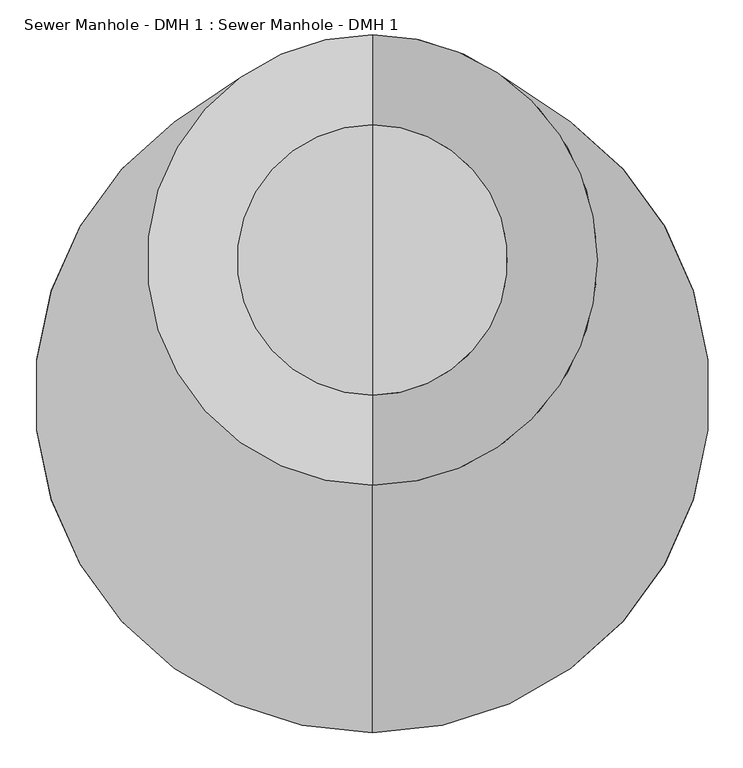
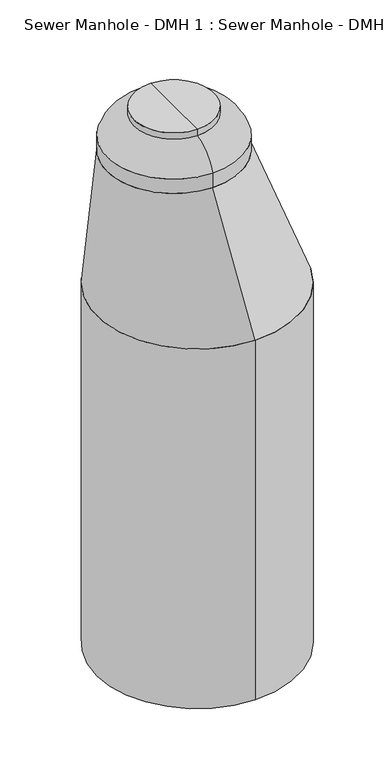
"""IFC4 building model written with IfcOpenShell, lengths in millimetres: proxy geometry, Sewer Manhole - DMH 1 : Sewer Manhole - DMH 1."""

from ifc_helpers import new_model, si_unit, point, frame, origin, place, context, project, spatial, circle_curve, ellipse_curve, trimmed, source, transform, mapped, element, save
from ifc_brep_helpers import plane_surface, cylinder_surface, revolved_surface, spline_surface, advanced_brep


def sewer_manhole_dmh_1_sewer_manhole_dmh_1_3a11640a(model_context):
    return source(origin(), model_context, "Body", "AdvancedBrep", [
        advanced_brep(
        [(0.0, -203.2, 3771.1270774), (0.0, 812.8, 3771.1270774), (0.0, -762.0, 2885.44), (0.0, 762.0, 2885.44)],
        [
            (0, 1, circle_curve(frame((0.0, 304.8, 3771.1270774), z_axis=(0.0, 0.0, 1.0), x_axis=(0.0, 1.0, 0.0)), 508.0)),
            (1, 0, circle_curve(frame((0.0, 304.8, 3771.1270774), z_axis=(0.0, 0.0, 1.0), x_axis=(0.0, 1.0, 0.0)), 508.0)),
            (2, 3, circle_curve(frame((0.0, 0.0, 2885.44), z_axis=(0.0, 0.0, -1.0), x_axis=(0.0, 1.0, 0.0)), 762.0)),
            (3, 2, circle_curve(frame((0.0, 0.0, 2885.44), z_axis=(0.0, 0.0, -1.0), x_axis=(0.0, 1.0, 0.0)), 762.0)),
            (3, 1),
            (0, 2),
        ],
        [
            plane_surface(frame((0.0, 304.8, 3771.1270774), z_axis=(0.0, 0.0, 1.0), x_axis=(1.0, 0.0, 0.0))),
            plane_surface(frame((0.0, 0.0, 2885.44), z_axis=(0.0, 0.0, -1.0), x_axis=(1.0, 0.0, 0.0))),
            spline_surface(2, 1, [[(0.0, -762.0, 2885.44), (0.0, -203.2, 3771.1270774)], [(762.0, -762.0, 2885.44), (508.0, -203.2, 3771.1270774)], [(762.0, 0.0, 2885.44), (508.0, 304.8, 3771.1270774)], [(762.0, 762.0, 2885.44), (508.0, 812.8, 3771.1270774)], [(0.0, 762.0, 2885.44), (0.0, 812.8, 3771.1270774)]], [3, 2, 3], [2, 2], [0.0, 1.0, 2.0], [0.0, 1.0], weights=[[1.0, 1.0], [0.7071067811865476, 0.7071067811865476], [1.0, 1.0], [0.7071067811865476, 0.7071067811865476], [1.0, 1.0]]),
            spline_surface(2, 1, [[(0.0, 762.0, 2885.44), (0.0, 812.8, 3771.1270774)], [(-762.0, 762.0, 2885.44), (-507.99999999999994, 812.8, 3771.1270774)], [(-762.0, 0.0, 2885.44), (-507.99999999999994, 304.8, 3771.1270774)], [(-762.0, -762.0, 2885.44), (-507.99999999999994, -203.19999999999993, 3771.1270774)], [(0.0, -762.0, 2885.44), (0.0, -203.2, 3771.1270774)]], [3, 2, 3], [2, 2], [0.0, 1.0, 2.0], [0.0, 1.0], weights=[[1.0, 1.0], [0.7071067811865476, 0.7071067811865476], [1.0, 1.0], [0.7071067811865476, 0.7071067811865476], [1.0, 1.0]]),
        ],
        [
            (0, [[1, 2]]),
            (1, [[3, 4]]),
            (2, [[-4, 5, -1, 6]]),
            (3, [[-3, -6, -2, -5]]),
        ],
    ),
        advanced_brep(
        [(0.0, -203.2, 3771.1270774), (0.0, 812.8, 3771.1270774), (0.0, 304.8, 3771.1270774), (0.0, -203.2, 3886.2), (0.0, 812.8, 3886.2), (0.0, 0.0, 4064.0), (0.0, 609.6, 4064.0), (0.0, 0.0, 4114.8), (0.0, 609.6, 4114.8), (0.0, 304.8, 4114.8)],
        [
            (0, 1, circle_curve(frame((0.0, 304.8, 3771.1270774), z_axis=(0.0, 0.0, -1.0), x_axis=(0.0, 1.0, 0.0)), 508.0)),
            (1, 2),
            (2, 0),
            (1, 0, circle_curve(frame((0.0, 304.8, 3771.1270774), z_axis=(0.0, 0.0, -1.0), x_axis=(0.0, 1.0, 0.0)), 508.0)),
            (3, 4, circle_curve(frame((0.0, 304.8, 3886.2), z_axis=(0.0, 0.0, -1.0), x_axis=(0.0, 1.0, 0.0)), 508.0)),
            (4, 1),
            (0, 3),
            (4, 3, circle_curve(frame((0.0, 304.8, 3886.2), z_axis=(0.0, 0.0, -1.0), x_axis=(0.0, 1.0, 0.0)), 508.0)),
            (5, 6, circle_curve(frame((0.0, 304.8, 4064.0), z_axis=(0.0, 0.0, -1.0), x_axis=(0.0, 1.0, 0.0)), 304.8)),
            (6, 4, circle_curve(frame((0.0, 564.4539436, 3807.3902213), z_axis=(-1.0, 0.0, 0.0), x_axis=(0.0, -1.0, 0.0)), 260.550849)),
            (3, 5, circle_curve(frame((0.0, 45.1460564, 3807.3902213), z_axis=(-1.0, 0.0, 0.0), x_axis=(0.0, 1.0, 0.0)), 260.550849)),
            (6, 5, circle_curve(frame((0.0, 304.8, 4064.0), z_axis=(0.0, 0.0, -1.0), x_axis=(0.0, 1.0, 0.0)), 304.8)),
            (7, 8, circle_curve(frame((0.0, 304.8, 4114.8), z_axis=(0.0, 0.0, -1.0), x_axis=(0.0, 1.0, 0.0)), 304.8)),
            (8, 6),
            (5, 7),
            (8, 7, circle_curve(frame((0.0, 304.8, 4114.8), z_axis=(0.0, 0.0, -1.0), x_axis=(0.0, 1.0, 0.0)), 304.8)),
            (9, 8),
            (7, 9),
        ],
        [
            plane_surface(frame((0.0, 304.8, 3771.1270774), z_axis=(0.0, 0.0, -1.0), x_axis=(0.0, 1.0, 0.0))),
            cylinder_surface(frame((0.0, 304.8, 3835.4), z_axis=(0.0, 0.0, 1.0), x_axis=(0.0, 1.0, 0.0)), 508.0),
            revolved_surface(trimmed(ellipse_curve(frame((0.0, 564.4539436, 3807.3902213), z_axis=(1.0, 0.0, 0.0), x_axis=(0.0, -1.0, 0.0)), 260.550849, 260.550849), [point((0.0, 812.8, 3886.2))], [point((0.0, 609.6, 4064.0))], True, "CARTESIAN"), (0.0, 304.8, 3835.4), (0.0, 0.0, 1.0)),
            cylinder_surface(frame((0.0, 304.8, 3835.4), z_axis=(0.0, 0.0, 1.0), x_axis=(0.0, 1.0, 0.0)), 304.8),
            plane_surface(frame((0.0, 304.8, 4114.8), z_axis=(0.0, 0.0, 1.0), x_axis=(0.0, 1.0, 0.0))),
        ],
        [
            (0, [[1, 2, 3]]),
            (0, [[4, -3, -2]]),
            (1, [[5, 6, -1, 7]]),
            (1, [[8, -7, -4, -6]]),
            (2, [[9, 10, -5, 11]]),
            (2, [[12, -11, -8, -10]]),
            (3, [[13, 14, -9, 15]]),
            (3, [[16, -15, -12, -14]]),
            (4, [[17, -13, 18]]),
            (4, [[-18, -16, -17]]),
        ],
    ),
        advanced_brep(
        [(0.0, -762.0, 2885.44), (0.0, 762.0, 2885.44), (0.0, 762.0, 0.0), (0.0, -762.0, 0.0), (0.0, 0.0, 0.0), (0.0, 0.0, 2885.44)],
        [
            (0, 1, circle_curve(frame((0.0, 0.0, 2885.44), z_axis=(0.0, 0.0, -1.0), x_axis=(0.0, 1.0, 0.0)), 762.0)),
            (1, 2),
            (2, 3, circle_curve(frame((0.0, 0.0, 0.0), z_axis=(0.0, 0.0, 1.0), x_axis=(0.0, 1.0, 0.0)), 762.0)),
            (3, 0),
            (1, 0, circle_curve(frame((0.0, 0.0, 2885.44), z_axis=(0.0, 0.0, -1.0), x_axis=(0.0, 1.0, 0.0)), 762.0)),
            (3, 2, circle_curve(frame((0.0, 0.0, 0.0), z_axis=(0.0, 0.0, 1.0), x_axis=(0.0, 1.0, 0.0)), 762.0)),
            (2, 4),
            (4, 3),
            (5, 1),
            (0, 5),
        ],
        [
            cylinder_surface(frame((0.0, 0.0, 457.2), z_axis=(0.0, 0.0, 1.0), x_axis=(0.0, 1.0, 0.0)), 762.0),
            plane_surface(frame((0.0, 0.0, 0.0), z_axis=(0.0, 0.0, -1.0), x_axis=(0.0, 1.0, 0.0))),
            plane_surface(frame((0.0, 0.0, 2885.44), z_axis=(0.0, 0.0, 1.0), x_axis=(0.0, 1.0, 0.0))),
        ],
        [
            (0, [[1, 2, 3, 4]]),
            (0, [[5, -4, 6, -2]]),
            (1, [[-3, 7, 8]]),
            (1, [[-6, -8, -7]]),
            (2, [[9, -1, 10]]),
            (2, [[-10, -5, -9]]),
        ],
    ),
    ])


if __name__ == "__main__":
    model = new_model("IFC4")
    model_context = context("Model", 3, world=origin())
    ifc_project = project(units=[si_unit("LENGTHUNIT", "METRE", prefix="MILLI")], contexts=[model_context])
    site = spatial("IfcSite", under=ifc_project)
    building = spatial("IfcBuilding", under=site)
    placement = place(None, origin())
    sewer_manhole_dmh_1_sewer_manhole_dmh_1_shape = sewer_manhole_dmh_1_sewer_manhole_dmh_1_3a11640a(model_context)
    element("IfcBuildingElementProxy", 1, Name="Sewer Manhole - DMH 1 : Sewer Manhole - DMH 1", ObjectType="Sewer Manhole - DMH 1 : Sewer Manhole - DMH 1", at=placement, inside=building, context=model_context, shape_type="MappedRepresentation", body=[
        mapped(sewer_manhole_dmh_1_sewer_manhole_dmh_1_shape, transform((0.0, 0.0, 0.0), x_axis=(1.0, 0.0, 0.0), y_axis=(0.0, 1.0, 0.0), z_axis=(0.0, 0.0, 1.0))),
    ])
    save(model, "model.ifc")
